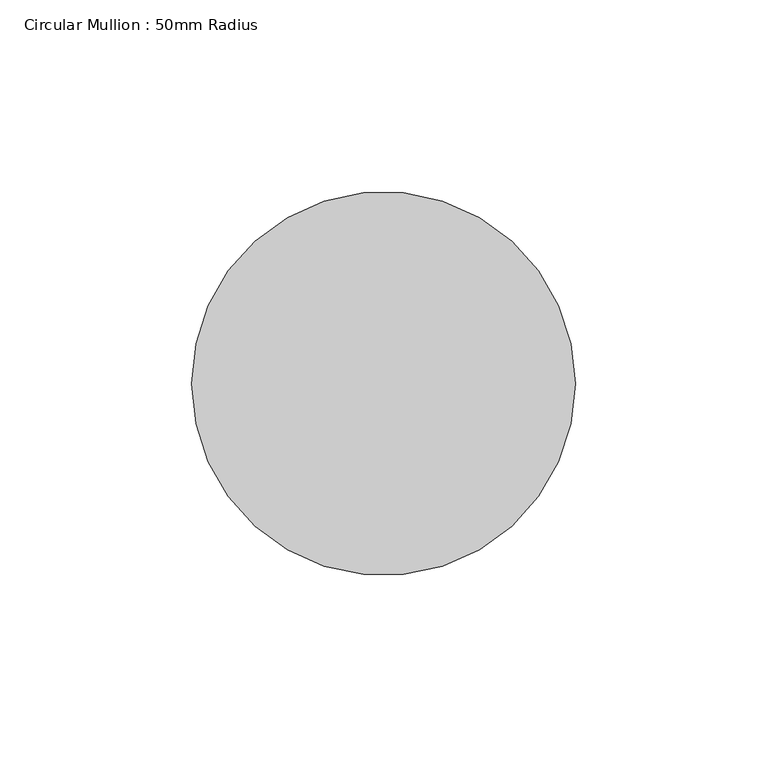
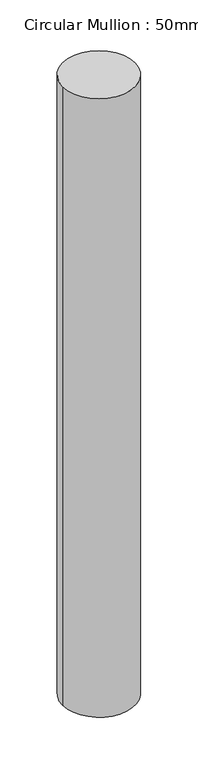
"""IFC4 building model written with IfcOpenShell, lengths in millimetres: member geometry, Circular Mullion : 50mm Radius."""

from ifc_helpers import new_model, si_unit, point, frame, origin, origin_2d, place, context, project, spatial, circle_curve, trimmed, segment, composite_curve, outline, extrude, source, transform, mapped, element, save


def circular_mullion_50mm_radius_bde59469(model_context):
    return source(origin(), model_context, "Body", "SweptSolid", [
        extrude(outline(composite_curve([segment(trimmed(circle_curve(origin_2d(), 50.0), [point((50.0, 0.0))], [point((-50.0, 0.0))], False, "CARTESIAN"), True, "CONTINUOUS"), segment(trimmed(circle_curve(origin_2d(), 50.0), [point((-50.0, 0.0))], [point((50.0, 0.0))], False, "CARTESIAN"), True, "CONTINUOUS")], self_intersect=False)), frame((0.0, 0.0, -901.1925426), z_axis=(0.0, 0.0, 1.0), x_axis=(1.0, 0.0, 0.0)), (0.0, 0.0, 1.0), 901.1925426),
    ])


if __name__ == "__main__":
    model = new_model("IFC4")
    model_context = context("Model", 3, world=origin())
    ifc_project = project(units=[si_unit("LENGTHUNIT", "METRE", prefix="MILLI")], contexts=[model_context])
    site = spatial("IfcSite", under=ifc_project)
    building = spatial("IfcBuilding", under=site)
    placement = place(None, origin())
    circular_mullion_50mm_radius_shape = circular_mullion_50mm_radius_bde59469(model_context)
    element("IfcMember", 1, ObjectType="Circular Mullion : 50mm Radius", at=placement, inside=building, context=model_context, shape_type="MappedRepresentation", body=[
        mapped(circular_mullion_50mm_radius_shape, transform((0.0, 0.0, 0.0), x_axis=(1.0, 0.0, 0.0), y_axis=(0.0, 1.0, 0.0), z_axis=(0.0, 0.0, 1.0))),
    ])
    save(model, "model.ifc")

# Revit data of these elements
# Type "Circular Mullion : 50mm Radius"
#   built-in parameter 1007350 = 0.164042 (stored number, unit not read)
# Element 1 (IfcMember, "Circular Mullion : 50mm Radius")
#   Materials on its faces: "Aluminium"
# Materials
#   "Aluminium": class "Metal", colour RGB 247 247 247, transparency 0, Description = "Aluminium 6061", Cost = 0
